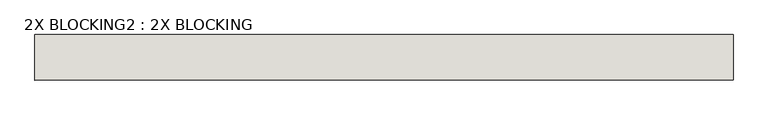
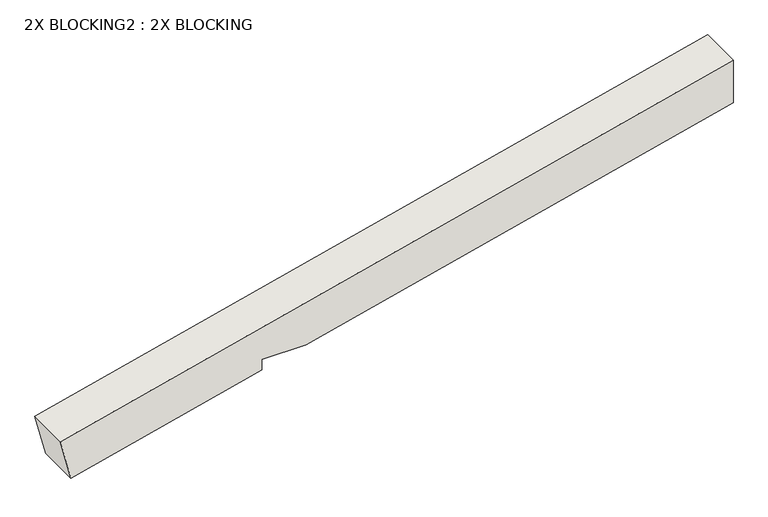
"""IFC4 building model written with IfcOpenShell, lengths in millimetres: wall geometry, 2X BLOCKING2 : 2X BLOCKING."""

from ifc_helpers import new_model, si_unit, frame, origin, place, context, project, spatial, polyline, outline, extrude, source, transform, mapped, element, save


def wall_2x_blocking2_2x_blocking_a19d3a84(model_context):
    return source(origin(), model_context, "Body", "SweptSolid", [
        extrude(outline(polyline([(2251.5843047, 17465.324224), (2403.475, 18072.8870052), (2438.4, 18072.8870052), (2438.4, 18212.5870052), (2778.125, 19571.4870052), (2922.124464, 19571.4870052), (2387.1346448, 17431.5277285), (2251.5843047, 17465.324224)])), frame((0.0, -1256.0384634, 0.0), z_axis=(0.0, 1.0, 0.0), x_axis=(0.0, 0.0, 1.0)), (0.0, 0.0, 1.0), 139.7),
    ])


if __name__ == "__main__":
    model = new_model("IFC4")
    model_context = context("Model", 3, world=origin())
    ifc_project = project(units=[si_unit("LENGTHUNIT", "METRE", prefix="MILLI")], contexts=[model_context])
    site = spatial("IfcSite", under=ifc_project)
    building = spatial("IfcBuilding", under=site)
    placement = place(None, origin())
    wall_2x_blocking2_2x_blocking_shape = wall_2x_blocking2_2x_blocking_a19d3a84(model_context)
    element("IfcWall", 1, ObjectType="2X BLOCKING2 : 2X BLOCKING", at=placement, inside=building, context=model_context, shape_type="MappedRepresentation", body=[
        mapped(wall_2x_blocking2_2x_blocking_shape, transform((0.0, 0.0, 0.0), x_axis=(1.0, 0.0, 0.0), y_axis=(0.0, 1.0, 0.0), z_axis=(0.0, 0.0, 1.0))),
    ])
    save(model, "model.ifc")

# Revit data of these elements
# Type "2X BLOCKING2 : 2X BLOCKING"
#   Structural Material = 2 X BLOCKING
# Element 1 (IfcWall, "2X BLOCKING2 : 2X BLOCKING")
#   Materials on its faces: "2 X 6 RAFTER BEYOND"
# Materials
#   "2 X BLOCKING": class "Wood", colour RGB 234 198 147, transparency 0, Description = "Pinus Echinata", Cost = 0
#   "2 X 6 RAFTER BEYOND": class "Wood", colour RGB 234 198 147, transparency 0, Description = "Pinus Echinata", Cost = 0
